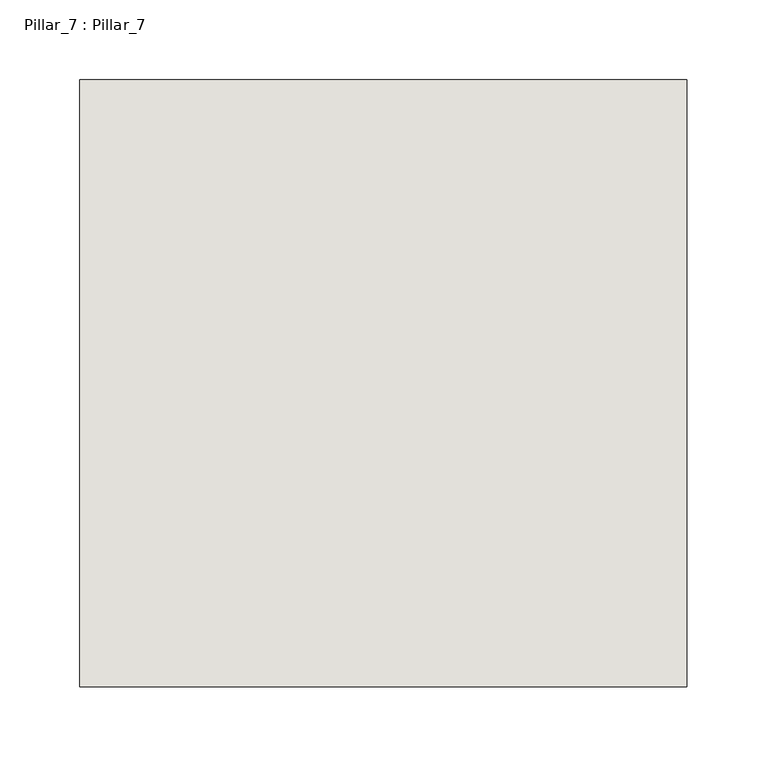
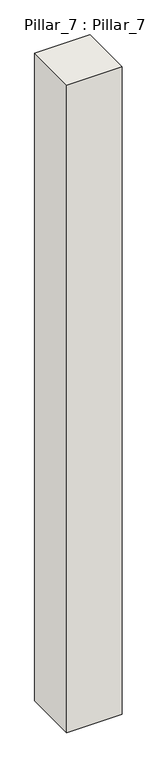
"""IFC4 building model written with IfcOpenShell, lengths in millimetres: wall geometry, Pillar_7 : Pillar_7."""

from ifc_helpers import new_model, si_unit, origin, origin_with_axes, place, context, project, spatial, polyline, outline, extrude, source, transform, mapped, element, save


def pillar_7_pillar_7_9e6fd231(model_context):
    return source(origin(), model_context, "Body", "SweptSolid", [
        extrude(outline(polyline([(3840.0, 15700.0), (3460.0, 15700.0), (3460.0, 16080.0), (3840.0, 16080.0), (3840.0, 15700.0)])), origin_with_axes(), (0.0, 0.0, 1.0), 4700.0),
    ])


if __name__ == "__main__":
    model = new_model("IFC4")
    model_context = context("Model", 3, world=origin())
    ifc_project = project(units=[si_unit("LENGTHUNIT", "METRE", prefix="MILLI")], contexts=[model_context])
    site = spatial("IfcSite", under=ifc_project)
    building = spatial("IfcBuilding", under=site)
    placement = place(None, origin())
    pillar_7_pillar_7_shape = pillar_7_pillar_7_9e6fd231(model_context)
    element("IfcWall", 1, ObjectType="Pillar_7 : Pillar_7", at=placement, inside=building, context=model_context, shape_type="MappedRepresentation", body=[
        mapped(pillar_7_pillar_7_shape, transform((0.0, 0.0, 0.0), x_axis=(1.0, 0.0, 0.0), y_axis=(0.0, 1.0, 0.0), z_axis=(0.0, 0.0, 1.0))),
    ])
    save(model, "model.ifc")

# Revit data of these elements
# Type "Pillar_7 : Pillar_7"
#   NameOverride = "Pillar_7"
# Element 1 (IfcWall, "Pillar_7 : Pillar_7")
#   Materials on its faces: "IfcSurfaceStyle #33"
# Materials
#   "IfcSurfaceStyle #33": class "Unassigned", colour RGB 214 214 214, transparency 0
